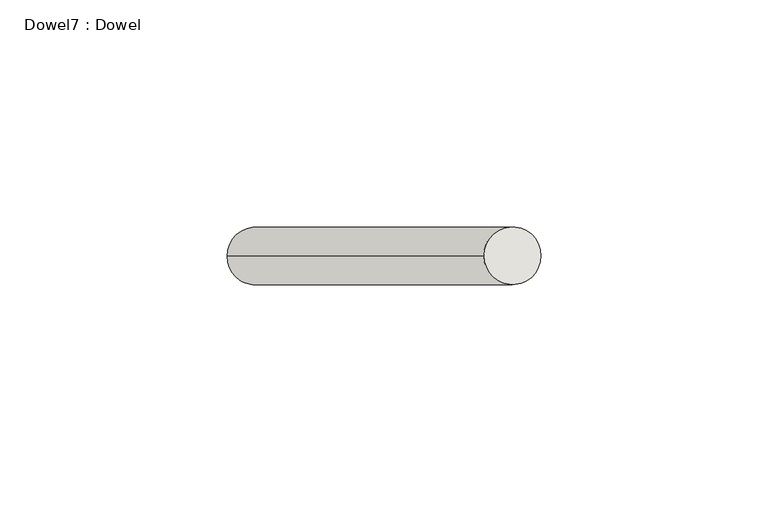
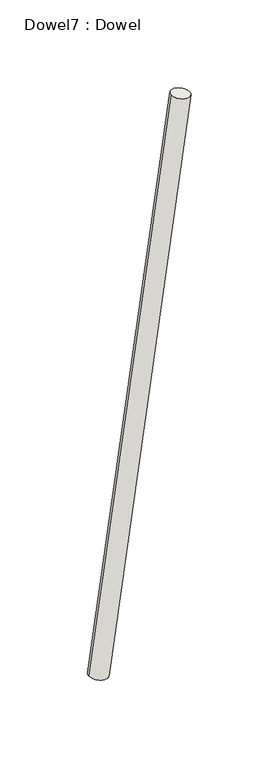
"""IFC4 building model written with IfcOpenShell, lengths in millimetres: wall geometry, Dowel7 : Dowel."""

import ifcopenshell
import ifcopenshell.guid

model = None  # the IFC model being written
_history = None  # IfcOwnerHistory: only IFC2X3 demands one
_inside = {}  # id of a spatial element -> (the spatial element, [elements in it])
_under = {}  # id of a project, library or spatial element -> (it, [spatial elements below it])
_declared = {}  # id of a project -> (the project, [libraries it declares])
_typed = {}  # id of a type object -> (the type object, [elements of that type])
_made_of = {}  # id of a material, layer set ... -> (it, [elements and type objects made of it])


def new_model(schema):
    """Start an empty IFC model of exactly this schema.

    Asked for "IFC4X3", IfcOpenShell would pick the latest addendum, in which some entities
    have other attributes; the version numbers below select the first issue.
    IFC2X3 requires an IfcOwnerHistory on every rooted entity: one is made here for all.
    """
    global model, _history
    if schema == "IFC4X3":
        model = ifcopenshell.file(schema_version=(4, 3, 0, 0))
    else:
        model = ifcopenshell.file(schema=schema)
    _inside.clear()
    _under.clear()
    _declared.clear()
    _typed.clear()
    _made_of.clear()
    _history = None
    if model.schema == "IFC2X3":
        org = make("IfcOrganization", Name="unknown")
        user = make(
            "IfcPersonAndOrganization",
            ThePerson=make("IfcPerson", FamilyName="unknown"),
            TheOrganization=org,
        )
        app = make(
            "IfcApplication",
            ApplicationDeveloper=org,
            Version="unknown",
            ApplicationFullName="unknown",
            ApplicationIdentifier="unknown",
        )
        _history = make(
            "IfcOwnerHistory",
            OwningUser=user,
            OwningApplication=app,
            ChangeAction="ADDED",
            CreationDate=0,
        )
    return model


def make(cls, **values):
    """One entity of the class cls with the attributes given. An attribute that is None is left unset."""
    return model.create_entity(
        cls, **{name: value for name, value in values.items() if value is not None}
    )


def rooted(cls, **values):
    """An entity with a GlobalId (a new one), such as an element, a storey or a relation."""
    return make(cls, GlobalId=ifcopenshell.guid.new(), OwnerHistory=_history, **values)


def si_unit(unit_type, name, prefix=None):
    """IfcSIUnit, for example si_unit("LENGTHUNIT", "METRE", prefix="MILLI")."""
    return make("IfcSIUnit", UnitType=unit_type, Prefix=prefix, Name=name)


def assignment(units):
    """IfcUnitAssignment: the units of a project."""
    return None if units is None else make("IfcUnitAssignment", Units=units)


def point(xyz):
    """IfcCartesianPoint."""
    return None if xyz is None else make("IfcCartesianPoint", Coordinates=xyz)


def direction(xyz):
    """IfcDirection."""
    return None if xyz is None else make("IfcDirection", DirectionRatios=xyz)


def frame(location, z_axis=None, x_axis=None):
    """IfcAxis2Placement3D, a coordinate frame: its origin and axes. An axis left out is left unset."""
    return make(
        "IfcAxis2Placement3D",
        Location=point(location),
        Axis=direction(z_axis),
        RefDirection=direction(x_axis),
    )


def frame_2d(location, x_axis=None):
    """IfcAxis2Placement2D, a coordinate frame in the plane: its origin and x axis."""
    return make(
        "IfcAxis2Placement2D", Location=point(location), RefDirection=direction(x_axis)
    )


def origin():
    """The frame at (0, 0, 0) with its axes left unset."""
    return frame((0.0, 0.0, 0.0))


def origin_2d():
    """The frame at (0, 0) in the plane with its x axis left unset."""
    return frame_2d((0.0, 0.0))


def place(relative_to, where):
    """IfcLocalPlacement: puts the frame where relative to a parent placement (None: the world)."""
    return make(
        "IfcLocalPlacement", PlacementRelTo=relative_to, RelativePlacement=where
    )


def context(
    kind, dimensions, precision=None, world=None, true_north=None, identifier=None
):
    """IfcGeometricRepresentationContext, for example the 3D "Model" context."""
    return make(
        "IfcGeometricRepresentationContext",
        ContextIdentifier=identifier,
        ContextType=kind,
        CoordinateSpaceDimension=dimensions,
        Precision=precision,
        WorldCoordinateSystem=world,
        TrueNorth=true_north,
    )


def project(units=None, contexts=None):
    """IfcProject with its units and contexts."""
    return rooted(
        "IfcProject",
        Name="project",
        RepresentationContexts=contexts,
        UnitsInContext=assignment(units),
    )


def spatial(cls, under=None, at=None, **own):
    """A site, building, storey or space (cls), placed at a placement, below another one or the project."""
    s = rooted(cls, ObjectPlacement=at, **own)
    if under is not None:
        _under.setdefault(under.id(), (under, []))[1].append(s)
    return s


def circle_curve(where, radius):
    """IfcCircle in the frame where."""
    return make("IfcCircle", Position=where, Radius=radius)


def trimmed(basis, trim1, trim2, sense, master):
    """IfcTrimmedCurve: the piece of a basis curve between two trims."""
    return make(
        "IfcTrimmedCurve",
        BasisCurve=basis,
        Trim1=trim1,
        Trim2=trim2,
        SenseAgreement=sense,
        MasterRepresentation=master,
    )


def segment(curve, same_sense, transition):
    """IfcCompositeCurveSegment."""
    return make(
        "IfcCompositeCurveSegment",
        Transition=transition,
        SameSense=same_sense,
        ParentCurve=curve,
    )


def composite_curve(segments, self_intersect=None):
    """IfcCompositeCurve: segments joined end to end."""
    return make("IfcCompositeCurve", Segments=segments, SelfIntersect=self_intersect)


def outline(outer, holes=None, kind="AREA"):
    """IfcArbitraryClosedProfileDef: a profile drawn as a closed curve; with holes, ...WithVoids."""
    if holes is None:
        return make("IfcArbitraryClosedProfileDef", ProfileType=kind, OuterCurve=outer)
    return make(
        "IfcArbitraryProfileDefWithVoids",
        ProfileType=kind,
        OuterCurve=outer,
        InnerCurves=holes,
    )


def extrude(swept, where, along, depth):
    """IfcExtrudedAreaSolid: the profile swept, set in the frame where, extruded along a direction by depth."""
    return make(
        "IfcExtrudedAreaSolid",
        SweptArea=swept,
        Position=where,
        ExtrudedDirection=direction(along),
        Depth=depth,
    )


def shape(context_of_items, identifier, shape_type, items):
    """IfcShapeRepresentation: the items that make up one representation, for example the "Body"."""
    return make(
        "IfcShapeRepresentation",
        ContextOfItems=context_of_items,
        RepresentationIdentifier=identifier,
        RepresentationType=shape_type,
        Items=items,
    )


def source(mapping_origin, context_of_items, identifier, shape_type, items):
    """IfcRepresentationMap: a shape defined once, which mapped items show again and again."""
    return make(
        "IfcRepresentationMap",
        MappingOrigin=mapping_origin,
        MappedRepresentation=shape(context_of_items, identifier, shape_type, items),
    )


def transform(
    local_origin,
    x_axis=None,
    y_axis=None,
    z_axis=None,
    scale=None,
    scale2=None,
    scale3=None,
    uniform=True,
):
    """IfcCartesianTransformationOperator3D, or its non-uniform kind. x_axis, y_axis, z_axis: its Axis1, 2, 3."""
    if uniform:
        return make(
            "IfcCartesianTransformationOperator3D",
            Axis1=direction(x_axis),
            Axis2=direction(y_axis),
            LocalOrigin=point(local_origin),
            Scale=scale,
            Axis3=direction(z_axis),
        )
    return make(
        "IfcCartesianTransformationOperator3DnonUniform",
        Axis1=direction(x_axis),
        Axis2=direction(y_axis),
        LocalOrigin=point(local_origin),
        Scale=scale,
        Axis3=direction(z_axis),
        Scale2=scale2,
        Scale3=scale3,
    )


def mapped(mapping_source, mapping_target):
    """IfcMappedItem: shows the shape of a source again, moved by a transform."""
    return make(
        "IfcMappedItem", MappingSource=mapping_source, MappingTarget=mapping_target
    )


def made_of(thing, what):
    """Note that an element or type object is made of a material, layer set ...; save() writes the relation."""
    if what is not None:
        _made_of.setdefault(what.id(), (what, []))[1].append(thing)
    return thing


def element(
    cls,
    number,
    at=None,
    inside=None,
    cuts=None,
    type_object=None,
    material=None,
    context=None,
    identifier="Body",
    shape_type=None,
    held_by="IfcProductDefinitionShape",
    body=None,
    shapes=None,
    **own,
):
    """One element of the class cls, such as IfcWall. Its Tag is "e" and its number.

    at: its placement. inside: the storey or other place that contains it. cuts: it is an
    opening in that element (IfcRelVoidsElement). A single representation is given by context,
    identifier, shape_type and body (its items); several are given by shapes. held_by: the class
    of the entity that holds the representations. save() writes the other relations.
    """
    e = rooted(cls, Tag="e%d" % number, ObjectPlacement=at, **own)
    if body is not None:
        shapes = [shape(context, identifier, shape_type, body)]
    if shapes is not None:
        e.Representation = make(held_by, Representations=shapes)
    if inside is not None:
        _inside.setdefault(inside.id(), (inside, []))[1].append(e)
    if cuts is not None:
        rooted(
            "IfcRelVoidsElement", RelatingBuildingElement=cuts, RelatedOpeningElement=e
        )
    if type_object is not None:
        _typed.setdefault(type_object.id(), (type_object, []))[1].append(e)
    return made_of(e, material)


def aggregate(whole, parts):
    """IfcRelAggregates: a whole, such as a stair, and the parts it consists of."""
    return rooted("IfcRelAggregates", RelatingObject=whole, RelatedObjects=parts)


def save(model, path):
    """Write the relations noted so far, then the file.

    IfcRelAggregates (storeys below a building ...), IfcRelContainedInSpatialStructure (elements
    in a storey), IfcRelDefinesByType, IfcRelAssociatesMaterial and IfcRelDeclares: one each for
    every whole, place, type object, material and project.
    """
    for whole, parts in _under.values():
        aggregate(whole, parts)
    for where, things in _inside.values():
        rooted(
            "IfcRelContainedInSpatialStructure",
            RelatedElements=things,
            RelatingStructure=where,
        )
    for kind, things in _typed.values():
        rooted("IfcRelDefinesByType", RelatedObjects=things, RelatingType=kind)
    for what, things in _made_of.values():
        rooted("IfcRelAssociatesMaterial", RelatedObjects=things, RelatingMaterial=what)
    for by, libraries in _declared.values():
        rooted("IfcRelDeclares", RelatingContext=by, RelatedDefinitions=libraries)
    model.write(path)


def dowel7_dowel_7052e6d0(model_context):
    return source(origin(), model_context, "Body", "SweptSolid", [
        extrude(outline(composite_curve([segment(trimmed(circle_curve(origin_2d(), 6.35), [point((0.0, -6.35))], [point((0.0, 6.3500001))], False, "CARTESIAN"), True, "CONTINUOUS"), segment(trimmed(circle_curve(origin_2d(), 6.35), [point((0.0, 6.3500001))], [point((0.0, -6.35))], False, "CARTESIAN"), True, "CONTINUOUS")], self_intersect=False)), frame((376630.0293887, 446.88125, 2084.1139617), z_axis=(0.13917310096003221, 0.0, 0.990268068741575), x_axis=(0.0, -1.0, 0.0)), (0.0, 0.0, 1.0), 406.4),
    ])


if __name__ == "__main__":
    model = new_model("IFC4")
    model_context = context("Model", 3, world=origin())
    ifc_project = project(units=[si_unit("LENGTHUNIT", "METRE", prefix="MILLI")], contexts=[model_context])
    site = spatial("IfcSite", under=ifc_project)
    building = spatial("IfcBuilding", under=site)
    placement = place(None, origin())
    dowel7_dowel_shape = dowel7_dowel_7052e6d0(model_context)
    element("IfcWall", 1, ObjectType="Dowel7 : Dowel", at=placement, inside=building, context=model_context, shape_type="MappedRepresentation", body=[
        mapped(dowel7_dowel_shape, transform((0.0, 0.0, 0.0), x_axis=(1.0, 0.0, 0.0), y_axis=(0.0, 1.0, 0.0), z_axis=(0.0, 0.0, 1.0))),
    ])
    save(model, "model.ifc")

# Revit data of these elements
# Element 1 (IfcWall, "Dowel7 : Dowel")
#   Materials on its faces: "#4 x 16\" BAR @ 2-0\" O.C. MAX. DRILL THRU HOLLOWCORE OR KEYWAY & INTO CIP WALL W/ 4\" MIN. EMBED"
# Materials
#   "#4 x 16\" BAR @ 2-0\" O.C. MAX. DRILL THRU HOLLOWCORE OR KEYWAY & INTO CIP WALL W/ 4\" MIN. EMBED": class "Generic", colour RGB 255 255 255, transparency 0, Cost = 0
